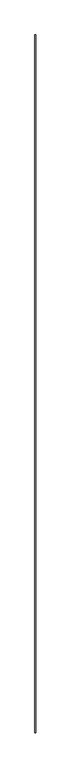
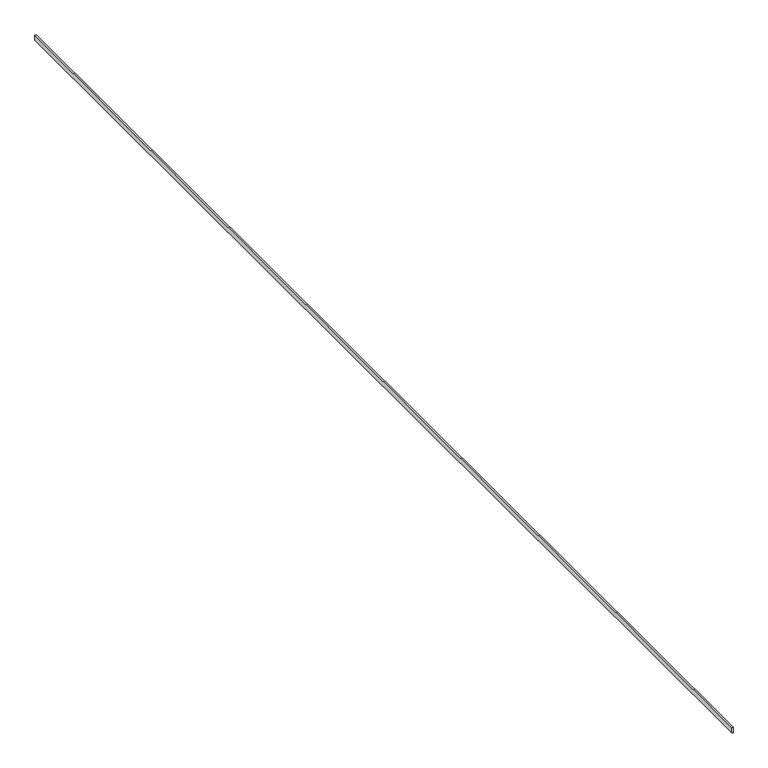
"""IFC4 building model written with IfcOpenShell, lengths in millimetres: proxy geometry, Generic Models 7:Generic Models 1:5:Generic Models 1:5 : Generic Models 7:Generic Models 1:337419:30 : Generic Models 7:Generic Models 1:5:Generic Models 1:5 : Generic Models 7:Generic Models 1:337419:311462."""

from ifc_helpers import new_model, si_unit, frame, origin, place, context, project, spatial, polyline, outline, extrude, source, transform, mapped, element, save


def generic_models_a10f0662(model_context):
    return source(origin(), model_context, "Body", "SweptSolid", [
        extrude(outline(polyline([(579326.7617241, -560020.541384), (579345.8117241, -560020.541384), (579345.8117239, -579008.999326), (579326.7617239, -579008.999326), (579326.7617241, -560020.541384)])), frame((0.0, 0.0, 4070.4332328), z_axis=(0.0, 0.0, 1.0), x_axis=(1.0, 0.0, 0.0)), (0.0, 0.0, 1.0), 86.2149083),
    ])


if __name__ == "__main__":
    model = new_model("IFC4")
    model_context = context("Model", 3, world=origin())
    ifc_project = project(units=[si_unit("LENGTHUNIT", "METRE", prefix="MILLI")], contexts=[model_context])
    site = spatial("IfcSite", under=ifc_project)
    building = spatial("IfcBuilding", under=site)
    placement = place(None, origin())
    generic_models_shape = generic_models_a10f0662(model_context)
    element("IfcBuildingElementProxy", 1, Name="Generic Models 7:Generic Models 1:5:Generic Models 1:5 : Generic Models 7:Generic Models 1:337419:30 : Generic Models 7:Generic Models 1:5:Generic Models 1:5 : Generic Models 7:Generic Models 1:337419:311462", ObjectType="Generic Models 7:Generic Models 1:5:Generic Models 1:5 : Generic Models 7:Generic Models 1:337419:30 : Generic Models 7:Generic Models 1:5:Generic Models 1:5 : Generic Models 7:Generic Models 1:337419:311462", at=placement, inside=building, context=model_context, shape_type="MappedRepresentation", body=[
        mapped(generic_models_shape, transform((0.0, 0.0, 0.0), x_axis=(1.0, 0.0, 0.0), y_axis=(0.0, 1.0, 0.0), z_axis=(0.0, 0.0, 1.0))),
    ])
    save(model, "model.ifc")

# Revit data of these elements
# Type "Generic Models 7:Generic Models 1:5:Generic Models 1:5 : Generic Models 7:Generic Models 1:337419:30 : Generic Models 7:Generic Models 1:5:Generic Models 1:5 : Generic Models 7:Generic Models 1:337419:311462"
#   NameOverride = "Generic Models 7:Generic Models 1:5:Generic Models 1:5 : Generic Models 7:Generic Models 1:337419:311462"
#   ObjectTypeOverride = "Generic Models 1:5 : Generic Models 7:Generic Models 1:337419"
#   Reference = "Generic Models 1"
#   Tag = "311462"
# Element 1 (IfcBuildingElementProxy, "Generic Models 7:Generic Models 1:5:Generic Models 1:5 : Generic Models 7:Generic Models 1:337419:30 : Generic Models 7:Generic Models 1:5:Generic Models 1:5 : Generic Models 7:Generic Models 1:337419:311462")
#   Materials on its faces: "1\" MINERAL WOOL BOARD INSULATION - BLACK MAT FACER"
# Materials
#   "1\" MINERAL WOOL BOARD INSULATION - BLACK MAT FACER": class "Unassigned", colour RGB 205 188 106, transparency 0, Cost = 0
